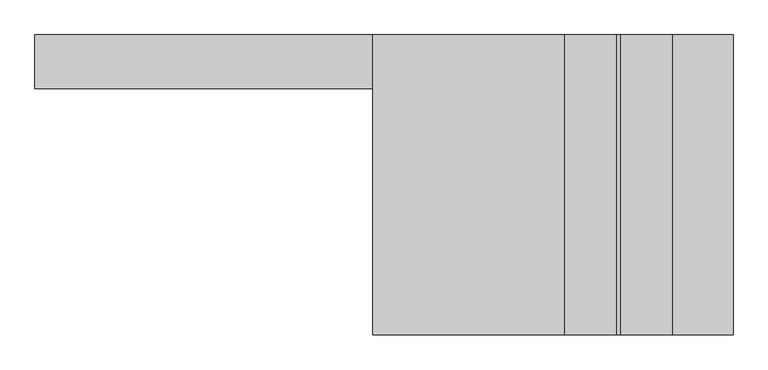
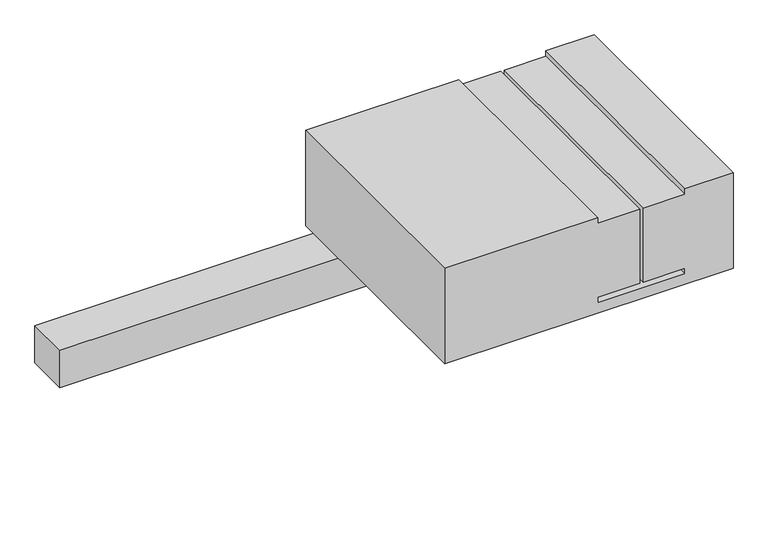
"""IFC4 building model written with IfcOpenShell, lengths in millimetres: proxy geometry, Framing058 2:Framing058 14884:298887 : Framing058 2:Framing058 14884:298887."""

import ifcopenshell
import ifcopenshell.guid

model = None  # the IFC model being written
_history = None  # IfcOwnerHistory: only IFC2X3 demands one
_inside = {}  # id of a spatial element -> (the spatial element, [elements in it])
_under = {}  # id of a project, library or spatial element -> (it, [spatial elements below it])
_declared = {}  # id of a project -> (the project, [libraries it declares])
_typed = {}  # id of a type object -> (the type object, [elements of that type])
_made_of = {}  # id of a material, layer set ... -> (it, [elements and type objects made of it])


def new_model(schema):
    """Start an empty IFC model of exactly this schema.

    Asked for "IFC4X3", IfcOpenShell would pick the latest addendum, in which some entities
    have other attributes; the version numbers below select the first issue.
    IFC2X3 requires an IfcOwnerHistory on every rooted entity: one is made here for all.
    """
    global model, _history
    if schema == "IFC4X3":
        model = ifcopenshell.file(schema_version=(4, 3, 0, 0))
    else:
        model = ifcopenshell.file(schema=schema)
    _inside.clear()
    _under.clear()
    _declared.clear()
    _typed.clear()
    _made_of.clear()
    _history = None
    if model.schema == "IFC2X3":
        org = make("IfcOrganization", Name="unknown")
        user = make(
            "IfcPersonAndOrganization",
            ThePerson=make("IfcPerson", FamilyName="unknown"),
            TheOrganization=org,
        )
        app = make(
            "IfcApplication",
            ApplicationDeveloper=org,
            Version="unknown",
            ApplicationFullName="unknown",
            ApplicationIdentifier="unknown",
        )
        _history = make(
            "IfcOwnerHistory",
            OwningUser=user,
            OwningApplication=app,
            ChangeAction="ADDED",
            CreationDate=0,
        )
    return model


def make(cls, **values):
    """One entity of the class cls with the attributes given. An attribute that is None is left unset."""
    return model.create_entity(
        cls, **{name: value for name, value in values.items() if value is not None}
    )


def rooted(cls, **values):
    """An entity with a GlobalId (a new one), such as an element, a storey or a relation."""
    return make(cls, GlobalId=ifcopenshell.guid.new(), OwnerHistory=_history, **values)


def si_unit(unit_type, name, prefix=None):
    """IfcSIUnit, for example si_unit("LENGTHUNIT", "METRE", prefix="MILLI")."""
    return make("IfcSIUnit", UnitType=unit_type, Prefix=prefix, Name=name)


def assignment(units):
    """IfcUnitAssignment: the units of a project."""
    return None if units is None else make("IfcUnitAssignment", Units=units)


def point(xyz):
    """IfcCartesianPoint."""
    return None if xyz is None else make("IfcCartesianPoint", Coordinates=xyz)


def direction(xyz):
    """IfcDirection."""
    return None if xyz is None else make("IfcDirection", DirectionRatios=xyz)


def frame(location, z_axis=None, x_axis=None):
    """IfcAxis2Placement3D, a coordinate frame: its origin and axes. An axis left out is left unset."""
    return make(
        "IfcAxis2Placement3D",
        Location=point(location),
        Axis=direction(z_axis),
        RefDirection=direction(x_axis),
    )


def origin():
    """The frame at (0, 0, 0) with its axes left unset."""
    return frame((0.0, 0.0, 0.0))


def place(relative_to, where):
    """IfcLocalPlacement: puts the frame where relative to a parent placement (None: the world)."""
    return make(
        "IfcLocalPlacement", PlacementRelTo=relative_to, RelativePlacement=where
    )


def context(
    kind, dimensions, precision=None, world=None, true_north=None, identifier=None
):
    """IfcGeometricRepresentationContext, for example the 3D "Model" context."""
    return make(
        "IfcGeometricRepresentationContext",
        ContextIdentifier=identifier,
        ContextType=kind,
        CoordinateSpaceDimension=dimensions,
        Precision=precision,
        WorldCoordinateSystem=world,
        TrueNorth=true_north,
    )


def project(units=None, contexts=None):
    """IfcProject with its units and contexts."""
    return rooted(
        "IfcProject",
        Name="project",
        RepresentationContexts=contexts,
        UnitsInContext=assignment(units),
    )


def spatial(cls, under=None, at=None, **own):
    """A site, building, storey or space (cls), placed at a placement, below another one or the project."""
    s = rooted(cls, ObjectPlacement=at, **own)
    if under is not None:
        _under.setdefault(under.id(), (under, []))[1].append(s)
    return s


def polyline(points):
    """IfcPolyline through the points."""
    return make("IfcPolyline", Points=[point(p) for p in points])


def outline(outer, holes=None, kind="AREA"):
    """IfcArbitraryClosedProfileDef: a profile drawn as a closed curve; with holes, ...WithVoids."""
    if holes is None:
        return make("IfcArbitraryClosedProfileDef", ProfileType=kind, OuterCurve=outer)
    return make(
        "IfcArbitraryProfileDefWithVoids",
        ProfileType=kind,
        OuterCurve=outer,
        InnerCurves=holes,
    )


def extrude(swept, where, along, depth):
    """IfcExtrudedAreaSolid: the profile swept, set in the frame where, extruded along a direction by depth."""
    return make(
        "IfcExtrudedAreaSolid",
        SweptArea=swept,
        Position=where,
        ExtrudedDirection=direction(along),
        Depth=depth,
    )


def shape(context_of_items, identifier, shape_type, items):
    """IfcShapeRepresentation: the items that make up one representation, for example the "Body"."""
    return make(
        "IfcShapeRepresentation",
        ContextOfItems=context_of_items,
        RepresentationIdentifier=identifier,
        RepresentationType=shape_type,
        Items=items,
    )


def source(mapping_origin, context_of_items, identifier, shape_type, items):
    """IfcRepresentationMap: a shape defined once, which mapped items show again and again."""
    return make(
        "IfcRepresentationMap",
        MappingOrigin=mapping_origin,
        MappedRepresentation=shape(context_of_items, identifier, shape_type, items),
    )


def transform(
    local_origin,
    x_axis=None,
    y_axis=None,
    z_axis=None,
    scale=None,
    scale2=None,
    scale3=None,
    uniform=True,
):
    """IfcCartesianTransformationOperator3D, or its non-uniform kind. x_axis, y_axis, z_axis: its Axis1, 2, 3."""
    if uniform:
        return make(
            "IfcCartesianTransformationOperator3D",
            Axis1=direction(x_axis),
            Axis2=direction(y_axis),
            LocalOrigin=point(local_origin),
            Scale=scale,
            Axis3=direction(z_axis),
        )
    return make(
        "IfcCartesianTransformationOperator3DnonUniform",
        Axis1=direction(x_axis),
        Axis2=direction(y_axis),
        LocalOrigin=point(local_origin),
        Scale=scale,
        Axis3=direction(z_axis),
        Scale2=scale2,
        Scale3=scale3,
    )


def mapped(mapping_source, mapping_target):
    """IfcMappedItem: shows the shape of a source again, moved by a transform."""
    return make(
        "IfcMappedItem", MappingSource=mapping_source, MappingTarget=mapping_target
    )


def made_of(thing, what):
    """Note that an element or type object is made of a material, layer set ...; save() writes the relation."""
    if what is not None:
        _made_of.setdefault(what.id(), (what, []))[1].append(thing)
    return thing


def element(
    cls,
    number,
    at=None,
    inside=None,
    cuts=None,
    type_object=None,
    material=None,
    context=None,
    identifier="Body",
    shape_type=None,
    held_by="IfcProductDefinitionShape",
    body=None,
    shapes=None,
    **own,
):
    """One element of the class cls, such as IfcWall. Its Tag is "e" and its number.

    at: its placement. inside: the storey or other place that contains it. cuts: it is an
    opening in that element (IfcRelVoidsElement). A single representation is given by context,
    identifier, shape_type and body (its items); several are given by shapes. held_by: the class
    of the entity that holds the representations. save() writes the other relations.
    """
    e = rooted(cls, Tag="e%d" % number, ObjectPlacement=at, **own)
    if body is not None:
        shapes = [shape(context, identifier, shape_type, body)]
    if shapes is not None:
        e.Representation = make(held_by, Representations=shapes)
    if inside is not None:
        _inside.setdefault(inside.id(), (inside, []))[1].append(e)
    if cuts is not None:
        rooted(
            "IfcRelVoidsElement", RelatingBuildingElement=cuts, RelatedOpeningElement=e
        )
    if type_object is not None:
        _typed.setdefault(type_object.id(), (type_object, []))[1].append(e)
    return made_of(e, material)


def aggregate(whole, parts):
    """IfcRelAggregates: a whole, such as a stair, and the parts it consists of."""
    return rooted("IfcRelAggregates", RelatingObject=whole, RelatedObjects=parts)


def save(model, path):
    """Write the relations noted so far, then the file.

    IfcRelAggregates (storeys below a building ...), IfcRelContainedInSpatialStructure (elements
    in a storey), IfcRelDefinesByType, IfcRelAssociatesMaterial and IfcRelDeclares: one each for
    every whole, place, type object, material and project.
    """
    for whole, parts in _under.values():
        aggregate(whole, parts)
    for where, things in _inside.values():
        rooted(
            "IfcRelContainedInSpatialStructure",
            RelatedElements=things,
            RelatingStructure=where,
        )
    for kind, things in _typed.values():
        rooted("IfcRelDefinesByType", RelatedObjects=things, RelatingType=kind)
    for what, things in _made_of.values():
        rooted("IfcRelAssociatesMaterial", RelatedObjects=things, RelatingMaterial=what)
    for by, libraries in _declared.values():
        rooted("IfcRelDeclares", RelatingContext=by, RelatedDefinitions=libraries)
    model.write(path)


def generic_models_ad19f543(model_context):
    return source(origin(), model_context, "Body", "SweptSolid", [
        extrude(outline(polyline([(4058.1226658, 1225.4418837), (4058.1226658, 1073.0418837), (2082.6354065, 1073.0418837), (2082.6354065, 1225.4418837), (4058.1226658, 1225.4418837)])), frame((0.0, 0.0, 39579.2960083), z_axis=(0.0, 0.0, 1.0), x_axis=(1.0, 0.0, 0.0)), (0.0, 0.0, 1.0), 139.7),
        extrude(outline(polyline([(39757.096, 3038.9476658), (39757.096, 4058.1226658), (40112.696, 4058.1226658), (40112.696, 3887.9426658), (40092.122, 3887.9426658), (40092.122, 3740.8131658), (39815.77, 3740.8131658), (39815.77, 3887.9426658), (39795.196, 3887.9426658), (39795.196, 3580.6026658), (39815.77, 3580.6026658), (39815.77, 3727.7321658), (40092.122, 3727.7321658), (40092.122, 3580.6026658), (40112.696, 3580.6026658), (40112.696, 3038.9476658), (39757.096, 3038.9476658)])), frame((0.0, 375.3200163, 0.0), z_axis=(0.0, 1.0, 0.0), x_axis=(0.0, 0.0, 1.0)), (0.0, 0.0, 1.0), 850.1218674),
    ])


if __name__ == "__main__":
    model = new_model("IFC4")
    model_context = context("Model", 3, world=origin())
    ifc_project = project(units=[si_unit("LENGTHUNIT", "METRE", prefix="MILLI")], contexts=[model_context])
    site = spatial("IfcSite", under=ifc_project)
    building = spatial("IfcBuilding", under=site)
    placement = place(None, origin())
    generic_models_shape = generic_models_ad19f543(model_context)
    element("IfcBuildingElementProxy", 1, Name="Framing058 2:Framing058 14884:298887 : Framing058 2:Framing058 14884:298887", ObjectType="Framing058 2:Framing058 14884:298887 : Framing058 2:Framing058 14884:298887", at=placement, inside=building, context=model_context, shape_type="MappedRepresentation", body=[
        mapped(generic_models_shape, transform((0.0, 0.0, 0.0), x_axis=(1.0, 0.0, 0.0), y_axis=(0.0, 1.0, 0.0), z_axis=(0.0, 0.0, 1.0))),
    ])
    save(model, "model.ifc")

# Revit data of these elements
# Type "Framing058 2:Framing058 14884:298887 : Framing058 2:Framing058 14884:298887"
#   NameOverride = "Framing058 2:Framing058 14884:298887"
#   ObjectTypeOverride = "Framing058 2:Framing058 14884"
#   Reference = "Framing058 14884"
#   Category = "Generic Models"
#   Tag = "298887"
# Element 1 (IfcBuildingElementProxy, "Framing058 2:Framing058 14884:298887 : Framing058 2:Framing058 14884:298887")
#   Materials on its faces: "WOOD FRAMING (SEE STRUCT DWGS)"
# Materials
#   "WOOD FRAMING (SEE STRUCT DWGS)": class "Unassigned", colour RGB 224 188 168, transparency 0, Cost = 0
